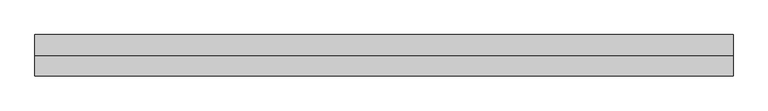
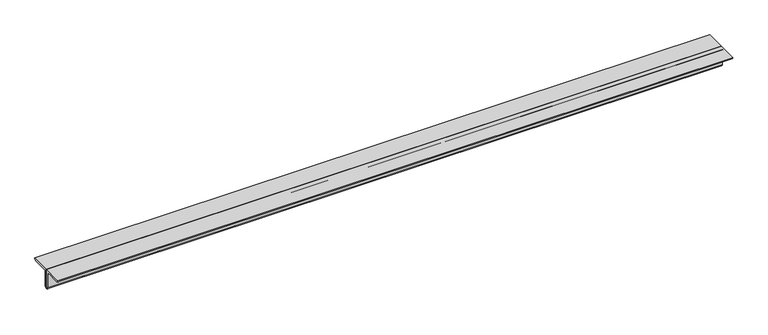
"""IFC4 building model written with IfcOpenShell, lengths in millimetres: member geometry, 0123_Steel Framing_2Ls-KSD3502 : H_SB_AR_S03_2Ls-130x130x12_HBR1."""

import ifcopenshell
import ifcopenshell.guid

model = None  # the IFC model being written
_history = None  # IfcOwnerHistory: only IFC2X3 demands one
_inside = {}  # id of a spatial element -> (the spatial element, [elements in it])
_under = {}  # id of a project, library or spatial element -> (it, [spatial elements below it])
_declared = {}  # id of a project -> (the project, [libraries it declares])
_typed = {}  # id of a type object -> (the type object, [elements of that type])
_made_of = {}  # id of a material, layer set ... -> (it, [elements and type objects made of it])


def new_model(schema):
    """Start an empty IFC model of exactly this schema.

    Asked for "IFC4X3", IfcOpenShell would pick the latest addendum, in which some entities
    have other attributes; the version numbers below select the first issue.
    IFC2X3 requires an IfcOwnerHistory on every rooted entity: one is made here for all.
    """
    global model, _history
    if schema == "IFC4X3":
        model = ifcopenshell.file(schema_version=(4, 3, 0, 0))
    else:
        model = ifcopenshell.file(schema=schema)
    _inside.clear()
    _under.clear()
    _declared.clear()
    _typed.clear()
    _made_of.clear()
    _history = None
    if model.schema == "IFC2X3":
        org = make("IfcOrganization", Name="unknown")
        user = make(
            "IfcPersonAndOrganization",
            ThePerson=make("IfcPerson", FamilyName="unknown"),
            TheOrganization=org,
        )
        app = make(
            "IfcApplication",
            ApplicationDeveloper=org,
            Version="unknown",
            ApplicationFullName="unknown",
            ApplicationIdentifier="unknown",
        )
        _history = make(
            "IfcOwnerHistory",
            OwningUser=user,
            OwningApplication=app,
            ChangeAction="ADDED",
            CreationDate=0,
        )
    return model


def make(cls, **values):
    """One entity of the class cls with the attributes given. An attribute that is None is left unset."""
    return model.create_entity(
        cls, **{name: value for name, value in values.items() if value is not None}
    )


def rooted(cls, **values):
    """An entity with a GlobalId (a new one), such as an element, a storey or a relation."""
    return make(cls, GlobalId=ifcopenshell.guid.new(), OwnerHistory=_history, **values)


def si_unit(unit_type, name, prefix=None):
    """IfcSIUnit, for example si_unit("LENGTHUNIT", "METRE", prefix="MILLI")."""
    return make("IfcSIUnit", UnitType=unit_type, Prefix=prefix, Name=name)


def assignment(units):
    """IfcUnitAssignment: the units of a project."""
    return None if units is None else make("IfcUnitAssignment", Units=units)


def point(xyz):
    """IfcCartesianPoint."""
    return None if xyz is None else make("IfcCartesianPoint", Coordinates=xyz)


def direction(xyz):
    """IfcDirection."""
    return None if xyz is None else make("IfcDirection", DirectionRatios=xyz)


def frame(location, z_axis=None, x_axis=None):
    """IfcAxis2Placement3D, a coordinate frame: its origin and axes. An axis left out is left unset."""
    return make(
        "IfcAxis2Placement3D",
        Location=point(location),
        Axis=direction(z_axis),
        RefDirection=direction(x_axis),
    )


def frame_2d(location, x_axis=None):
    """IfcAxis2Placement2D, a coordinate frame in the plane: its origin and x axis."""
    return make(
        "IfcAxis2Placement2D", Location=point(location), RefDirection=direction(x_axis)
    )


def origin():
    """The frame at (0, 0, 0) with its axes left unset."""
    return frame((0.0, 0.0, 0.0))


def place(relative_to, where):
    """IfcLocalPlacement: puts the frame where relative to a parent placement (None: the world)."""
    return make(
        "IfcLocalPlacement", PlacementRelTo=relative_to, RelativePlacement=where
    )


def context(
    kind, dimensions, precision=None, world=None, true_north=None, identifier=None
):
    """IfcGeometricRepresentationContext, for example the 3D "Model" context."""
    return make(
        "IfcGeometricRepresentationContext",
        ContextIdentifier=identifier,
        ContextType=kind,
        CoordinateSpaceDimension=dimensions,
        Precision=precision,
        WorldCoordinateSystem=world,
        TrueNorth=true_north,
    )


def project(units=None, contexts=None):
    """IfcProject with its units and contexts."""
    return rooted(
        "IfcProject",
        Name="project",
        RepresentationContexts=contexts,
        UnitsInContext=assignment(units),
    )


def spatial(cls, under=None, at=None, **own):
    """A site, building, storey or space (cls), placed at a placement, below another one or the project."""
    s = rooted(cls, ObjectPlacement=at, **own)
    if under is not None:
        _under.setdefault(under.id(), (under, []))[1].append(s)
    return s


def polyline(points):
    """IfcPolyline through the points."""
    return make("IfcPolyline", Points=[point(p) for p in points])


def circle_curve(where, radius):
    """IfcCircle in the frame where."""
    return make("IfcCircle", Position=where, Radius=radius)


def trimmed(basis, trim1, trim2, sense, master):
    """IfcTrimmedCurve: the piece of a basis curve between two trims."""
    return make(
        "IfcTrimmedCurve",
        BasisCurve=basis,
        Trim1=trim1,
        Trim2=trim2,
        SenseAgreement=sense,
        MasterRepresentation=master,
    )


def segment(curve, same_sense, transition):
    """IfcCompositeCurveSegment."""
    return make(
        "IfcCompositeCurveSegment",
        Transition=transition,
        SameSense=same_sense,
        ParentCurve=curve,
    )


def composite_curve(segments, self_intersect=None):
    """IfcCompositeCurve: segments joined end to end."""
    return make("IfcCompositeCurve", Segments=segments, SelfIntersect=self_intersect)


def outline(outer, holes=None, kind="AREA"):
    """IfcArbitraryClosedProfileDef: a profile drawn as a closed curve; with holes, ...WithVoids."""
    if holes is None:
        return make("IfcArbitraryClosedProfileDef", ProfileType=kind, OuterCurve=outer)
    return make(
        "IfcArbitraryProfileDefWithVoids",
        ProfileType=kind,
        OuterCurve=outer,
        InnerCurves=holes,
    )


def extrude(swept, where, along, depth):
    """IfcExtrudedAreaSolid: the profile swept, set in the frame where, extruded along a direction by depth."""
    return make(
        "IfcExtrudedAreaSolid",
        SweptArea=swept,
        Position=where,
        ExtrudedDirection=direction(along),
        Depth=depth,
    )


def shape(context_of_items, identifier, shape_type, items):
    """IfcShapeRepresentation: the items that make up one representation, for example the "Body"."""
    return make(
        "IfcShapeRepresentation",
        ContextOfItems=context_of_items,
        RepresentationIdentifier=identifier,
        RepresentationType=shape_type,
        Items=items,
    )


def source(mapping_origin, context_of_items, identifier, shape_type, items):
    """IfcRepresentationMap: a shape defined once, which mapped items show again and again."""
    return make(
        "IfcRepresentationMap",
        MappingOrigin=mapping_origin,
        MappedRepresentation=shape(context_of_items, identifier, shape_type, items),
    )


def transform(
    local_origin,
    x_axis=None,
    y_axis=None,
    z_axis=None,
    scale=None,
    scale2=None,
    scale3=None,
    uniform=True,
):
    """IfcCartesianTransformationOperator3D, or its non-uniform kind. x_axis, y_axis, z_axis: its Axis1, 2, 3."""
    if uniform:
        return make(
            "IfcCartesianTransformationOperator3D",
            Axis1=direction(x_axis),
            Axis2=direction(y_axis),
            LocalOrigin=point(local_origin),
            Scale=scale,
            Axis3=direction(z_axis),
        )
    return make(
        "IfcCartesianTransformationOperator3DnonUniform",
        Axis1=direction(x_axis),
        Axis2=direction(y_axis),
        LocalOrigin=point(local_origin),
        Scale=scale,
        Axis3=direction(z_axis),
        Scale2=scale2,
        Scale3=scale3,
    )


def mapped(mapping_source, mapping_target):
    """IfcMappedItem: shows the shape of a source again, moved by a transform."""
    return make(
        "IfcMappedItem", MappingSource=mapping_source, MappingTarget=mapping_target
    )


def made_of(thing, what):
    """Note that an element or type object is made of a material, layer set ...; save() writes the relation."""
    if what is not None:
        _made_of.setdefault(what.id(), (what, []))[1].append(thing)
    return thing


def element(
    cls,
    number,
    at=None,
    inside=None,
    cuts=None,
    type_object=None,
    material=None,
    context=None,
    identifier="Body",
    shape_type=None,
    held_by="IfcProductDefinitionShape",
    body=None,
    shapes=None,
    **own,
):
    """One element of the class cls, such as IfcWall. Its Tag is "e" and its number.

    at: its placement. inside: the storey or other place that contains it. cuts: it is an
    opening in that element (IfcRelVoidsElement). A single representation is given by context,
    identifier, shape_type and body (its items); several are given by shapes. held_by: the class
    of the entity that holds the representations. save() writes the other relations.
    """
    e = rooted(cls, Tag="e%d" % number, ObjectPlacement=at, **own)
    if body is not None:
        shapes = [shape(context, identifier, shape_type, body)]
    if shapes is not None:
        e.Representation = make(held_by, Representations=shapes)
    if inside is not None:
        _inside.setdefault(inside.id(), (inside, []))[1].append(e)
    if cuts is not None:
        rooted(
            "IfcRelVoidsElement", RelatingBuildingElement=cuts, RelatedOpeningElement=e
        )
    if type_object is not None:
        _typed.setdefault(type_object.id(), (type_object, []))[1].append(e)
    return made_of(e, material)


def aggregate(whole, parts):
    """IfcRelAggregates: a whole, such as a stair, and the parts it consists of."""
    return rooted("IfcRelAggregates", RelatingObject=whole, RelatedObjects=parts)


def save(model, path):
    """Write the relations noted so far, then the file.

    IfcRelAggregates (storeys below a building ...), IfcRelContainedInSpatialStructure (elements
    in a storey), IfcRelDefinesByType, IfcRelAssociatesMaterial and IfcRelDeclares: one each for
    every whole, place, type object, material and project.
    """
    for whole, parts in _under.values():
        aggregate(whole, parts)
    for where, things in _inside.values():
        rooted(
            "IfcRelContainedInSpatialStructure",
            RelatedElements=things,
            RelatingStructure=where,
        )
    for kind, things in _typed.values():
        rooted("IfcRelDefinesByType", RelatedObjects=things, RelatingType=kind)
    for what, things in _made_of.values():
        rooted("IfcRelAssociatesMaterial", RelatedObjects=things, RelatingMaterial=what)
    for by, libraries in _declared.values():
        rooted("IfcRelDeclares", RelatingContext=by, RelatedDefinitions=libraries)
    model.write(path)


def member_e19a7e3f(model_context):
    return source(origin(), model_context, "Body", "SweptSolid", [
        extrude(outline(composite_curve([segment(polyline([(0.0, 36.4), (130.0, 36.4)]), True, "CONTINUOUS"), segment(trimmed(circle_curve(frame_2d((118.0, 36.4)), 12.0), [point((130.0, 36.4))], [point((118.0, 24.4))], False, "CARTESIAN"), True, "CONTINUOUS"), segment(polyline([(118.0, 24.4), (24.0, 24.4)]), True, "CONTINUOUS"), segment(trimmed(circle_curve(frame_2d((24.0, 12.4)), 12.0), [point((24.0, 24.4))], [point((12.0, 12.4))], True, "CARTESIAN"), True, "CONTINUOUS"), segment(polyline([(12.0, 12.4), (12.0, -81.6)]), True, "CONTINUOUS"), segment(trimmed(circle_curve(frame_2d((0.0, -81.6)), 12.0), [point((12.0, -81.6))], [point((0.0, -93.6))], False, "CARTESIAN"), True, "CONTINUOUS"), segment(polyline([(0.0, -93.6), (0.0, 36.4)]), True, "CONTINUOUS")], self_intersect=False)), frame((-2158.4448527, 0.0, 0.0), z_axis=(1.0, 0.0, 0.0), x_axis=(0.0, 1.0, 0.0)), (0.0, 0.0, 1.0), 4391.0649986),
        extrude(outline(composite_curve([segment(polyline([(0.0, 36.4), (0.0, -93.6)]), True, "CONTINUOUS"), segment(trimmed(circle_curve(frame_2d((0.0, -81.6)), 12.0), [point((0.0, -93.6))], [point((-12.0, -81.6))], False, "CARTESIAN"), True, "CONTINUOUS"), segment(polyline([(-12.0, -81.6), (-12.0, 12.4)]), True, "CONTINUOUS"), segment(trimmed(circle_curve(frame_2d((-24.0, 12.4)), 12.0), [point((-12.0, 12.4))], [point((-24.0, 24.4))], True, "CARTESIAN"), True, "CONTINUOUS"), segment(polyline([(-24.0, 24.4), (-118.0, 24.4)]), True, "CONTINUOUS"), segment(trimmed(circle_curve(frame_2d((-118.0, 36.4)), 12.0), [point((-118.0, 24.4))], [point((-130.0, 36.4))], False, "CARTESIAN"), True, "CONTINUOUS"), segment(polyline([(-130.0, 36.4), (0.0, 36.4)]), True, "CONTINUOUS")], self_intersect=False)), frame((-2158.4448527, 0.0, 0.0), z_axis=(1.0, 0.0, 0.0), x_axis=(0.0, 1.0, 0.0)), (0.0, 0.0, 1.0), 4391.0649986),
    ])


if __name__ == "__main__":
    model = new_model("IFC4")
    model_context = context("Model", 3, world=origin())
    ifc_project = project(units=[si_unit("LENGTHUNIT", "METRE", prefix="MILLI")], contexts=[model_context])
    site = spatial("IfcSite", under=ifc_project)
    building = spatial("IfcBuilding", under=site)
    placement = place(None, origin())
    member_shape = member_e19a7e3f(model_context)
    element("IfcMember", 1, ObjectType="0123_Steel Framing_2Ls-KSD3502 : H_SB_AR_S03_2Ls-130x130x12_HBR1", at=placement, inside=building, context=model_context, shape_type="MappedRepresentation", body=[
        mapped(member_shape, transform((0.0, 0.0, 0.0), x_axis=(1.0, 0.0, 0.0), y_axis=(0.0, 1.0, 0.0), z_axis=(0.0, 0.0, 1.0))),
    ])
    save(model, "model.ifc")

# Revit data of these elements
# Type "0123_Steel Framing_2Ls-KSD3502 : H_SB_AR_S03_2Ls-130x130x12_HBR1"
#   Type Mark = "HBR1"
#   Assembly Code = "B10"
#   Legs = "SLBB"
#   W = 8.97
#   Perimeter = 1.04 m²/m
#   Nominal Weight = 46.80 kgf/m
#   Length [instance default] = 1000 mm
#   Space = 0 mm
#   b = 130 mm
#   d = 130 mm
#   t = 12 mm
#   y = 36.4 mm
#   A = 0.005952 m²
#   Structural Material [instance default] = Steel ASTM A36
# Element 1 (IfcMember, "0123_Steel Framing_2Ls-KSD3502 : H_SB_AR_S03_2Ls-130x130x12_HBR1")
#   Materials on its faces: "Steel ASTM A36"
# Materials
#   "Steel ASTM A36": class "Metal", colour RGB 199 199 199, transparency 0, Description = "Structural steel, ASTM A36 Grade B, mill finish", Cost = 0
